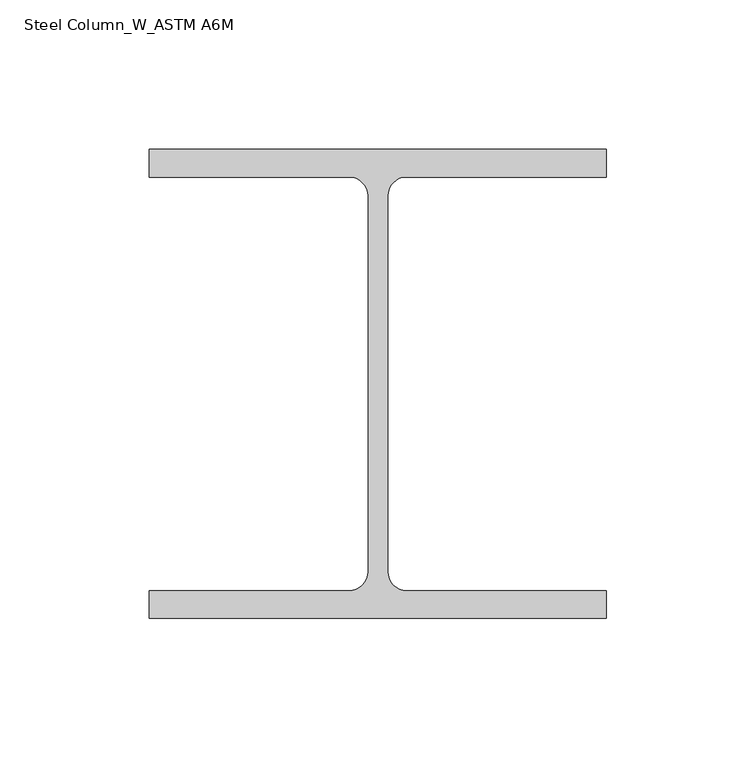
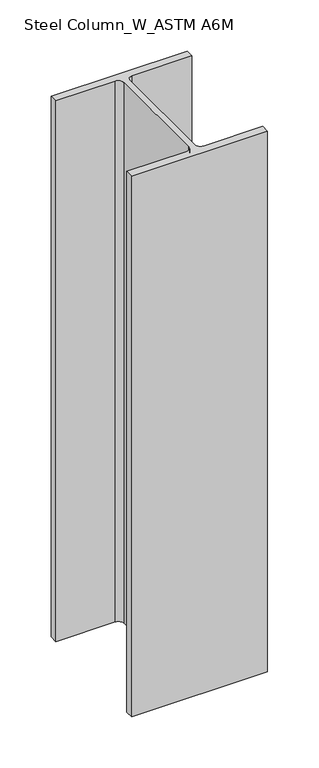
"""IFC4 building model written with IfcOpenShell, lengths in millimetres: column geometry, Steel Column_W_ASTM A6M : H_SC_AR_S01_W150x29.8_P1."""

import ifcopenshell
import ifcopenshell.guid

model = None  # the IFC model being written
_history = None  # IfcOwnerHistory: only IFC2X3 demands one
_inside = {}  # id of a spatial element -> (the spatial element, [elements in it])
_under = {}  # id of a project, library or spatial element -> (it, [spatial elements below it])
_declared = {}  # id of a project -> (the project, [libraries it declares])
_typed = {}  # id of a type object -> (the type object, [elements of that type])
_made_of = {}  # id of a material, layer set ... -> (it, [elements and type objects made of it])


def new_model(schema):
    """Start an empty IFC model of exactly this schema.

    Asked for "IFC4X3", IfcOpenShell would pick the latest addendum, in which some entities
    have other attributes; the version numbers below select the first issue.
    IFC2X3 requires an IfcOwnerHistory on every rooted entity: one is made here for all.
    """
    global model, _history
    if schema == "IFC4X3":
        model = ifcopenshell.file(schema_version=(4, 3, 0, 0))
    else:
        model = ifcopenshell.file(schema=schema)
    _inside.clear()
    _under.clear()
    _declared.clear()
    _typed.clear()
    _made_of.clear()
    _history = None
    if model.schema == "IFC2X3":
        org = make("IfcOrganization", Name="unknown")
        user = make(
            "IfcPersonAndOrganization",
            ThePerson=make("IfcPerson", FamilyName="unknown"),
            TheOrganization=org,
        )
        app = make(
            "IfcApplication",
            ApplicationDeveloper=org,
            Version="unknown",
            ApplicationFullName="unknown",
            ApplicationIdentifier="unknown",
        )
        _history = make(
            "IfcOwnerHistory",
            OwningUser=user,
            OwningApplication=app,
            ChangeAction="ADDED",
            CreationDate=0,
        )
    return model


def make(cls, **values):
    """One entity of the class cls with the attributes given. An attribute that is None is left unset."""
    return model.create_entity(
        cls, **{name: value for name, value in values.items() if value is not None}
    )


def rooted(cls, **values):
    """An entity with a GlobalId (a new one), such as an element, a storey or a relation."""
    return make(cls, GlobalId=ifcopenshell.guid.new(), OwnerHistory=_history, **values)


def si_unit(unit_type, name, prefix=None):
    """IfcSIUnit, for example si_unit("LENGTHUNIT", "METRE", prefix="MILLI")."""
    return make("IfcSIUnit", UnitType=unit_type, Prefix=prefix, Name=name)


def assignment(units):
    """IfcUnitAssignment: the units of a project."""
    return None if units is None else make("IfcUnitAssignment", Units=units)


def point(xyz):
    """IfcCartesianPoint."""
    return None if xyz is None else make("IfcCartesianPoint", Coordinates=xyz)


def direction(xyz):
    """IfcDirection."""
    return None if xyz is None else make("IfcDirection", DirectionRatios=xyz)


def frame(location, z_axis=None, x_axis=None):
    """IfcAxis2Placement3D, a coordinate frame: its origin and axes. An axis left out is left unset."""
    return make(
        "IfcAxis2Placement3D",
        Location=point(location),
        Axis=direction(z_axis),
        RefDirection=direction(x_axis),
    )


def frame_2d(location, x_axis=None):
    """IfcAxis2Placement2D, a coordinate frame in the plane: its origin and x axis."""
    return make(
        "IfcAxis2Placement2D", Location=point(location), RefDirection=direction(x_axis)
    )


def origin():
    """The frame at (0, 0, 0) with its axes left unset."""
    return frame((0.0, 0.0, 0.0))


def place(relative_to, where):
    """IfcLocalPlacement: puts the frame where relative to a parent placement (None: the world)."""
    return make(
        "IfcLocalPlacement", PlacementRelTo=relative_to, RelativePlacement=where
    )


def context(
    kind, dimensions, precision=None, world=None, true_north=None, identifier=None
):
    """IfcGeometricRepresentationContext, for example the 3D "Model" context."""
    return make(
        "IfcGeometricRepresentationContext",
        ContextIdentifier=identifier,
        ContextType=kind,
        CoordinateSpaceDimension=dimensions,
        Precision=precision,
        WorldCoordinateSystem=world,
        TrueNorth=true_north,
    )


def project(units=None, contexts=None):
    """IfcProject with its units and contexts."""
    return rooted(
        "IfcProject",
        Name="project",
        RepresentationContexts=contexts,
        UnitsInContext=assignment(units),
    )


def spatial(cls, under=None, at=None, **own):
    """A site, building, storey or space (cls), placed at a placement, below another one or the project."""
    s = rooted(cls, ObjectPlacement=at, **own)
    if under is not None:
        _under.setdefault(under.id(), (under, []))[1].append(s)
    return s


def polyline(points):
    """IfcPolyline through the points."""
    return make("IfcPolyline", Points=[point(p) for p in points])


def circle_curve(where, radius):
    """IfcCircle in the frame where."""
    return make("IfcCircle", Position=where, Radius=radius)


def trimmed(basis, trim1, trim2, sense, master):
    """IfcTrimmedCurve: the piece of a basis curve between two trims."""
    return make(
        "IfcTrimmedCurve",
        BasisCurve=basis,
        Trim1=trim1,
        Trim2=trim2,
        SenseAgreement=sense,
        MasterRepresentation=master,
    )


def segment(curve, same_sense, transition):
    """IfcCompositeCurveSegment."""
    return make(
        "IfcCompositeCurveSegment",
        Transition=transition,
        SameSense=same_sense,
        ParentCurve=curve,
    )


def composite_curve(segments, self_intersect=None):
    """IfcCompositeCurve: segments joined end to end."""
    return make("IfcCompositeCurve", Segments=segments, SelfIntersect=self_intersect)


def outline(outer, holes=None, kind="AREA"):
    """IfcArbitraryClosedProfileDef: a profile drawn as a closed curve; with holes, ...WithVoids."""
    if holes is None:
        return make("IfcArbitraryClosedProfileDef", ProfileType=kind, OuterCurve=outer)
    return make(
        "IfcArbitraryProfileDefWithVoids",
        ProfileType=kind,
        OuterCurve=outer,
        InnerCurves=holes,
    )


def extrude(swept, where, along, depth):
    """IfcExtrudedAreaSolid: the profile swept, set in the frame where, extruded along a direction by depth."""
    return make(
        "IfcExtrudedAreaSolid",
        SweptArea=swept,
        Position=where,
        ExtrudedDirection=direction(along),
        Depth=depth,
    )


def shape(context_of_items, identifier, shape_type, items):
    """IfcShapeRepresentation: the items that make up one representation, for example the "Body"."""
    return make(
        "IfcShapeRepresentation",
        ContextOfItems=context_of_items,
        RepresentationIdentifier=identifier,
        RepresentationType=shape_type,
        Items=items,
    )


def source(mapping_origin, context_of_items, identifier, shape_type, items):
    """IfcRepresentationMap: a shape defined once, which mapped items show again and again."""
    return make(
        "IfcRepresentationMap",
        MappingOrigin=mapping_origin,
        MappedRepresentation=shape(context_of_items, identifier, shape_type, items),
    )


def transform(
    local_origin,
    x_axis=None,
    y_axis=None,
    z_axis=None,
    scale=None,
    scale2=None,
    scale3=None,
    uniform=True,
):
    """IfcCartesianTransformationOperator3D, or its non-uniform kind. x_axis, y_axis, z_axis: its Axis1, 2, 3."""
    if uniform:
        return make(
            "IfcCartesianTransformationOperator3D",
            Axis1=direction(x_axis),
            Axis2=direction(y_axis),
            LocalOrigin=point(local_origin),
            Scale=scale,
            Axis3=direction(z_axis),
        )
    return make(
        "IfcCartesianTransformationOperator3DnonUniform",
        Axis1=direction(x_axis),
        Axis2=direction(y_axis),
        LocalOrigin=point(local_origin),
        Scale=scale,
        Axis3=direction(z_axis),
        Scale2=scale2,
        Scale3=scale3,
    )


def mapped(mapping_source, mapping_target):
    """IfcMappedItem: shows the shape of a source again, moved by a transform."""
    return make(
        "IfcMappedItem", MappingSource=mapping_source, MappingTarget=mapping_target
    )


def made_of(thing, what):
    """Note that an element or type object is made of a material, layer set ...; save() writes the relation."""
    if what is not None:
        _made_of.setdefault(what.id(), (what, []))[1].append(thing)
    return thing


def element(
    cls,
    number,
    at=None,
    inside=None,
    cuts=None,
    type_object=None,
    material=None,
    context=None,
    identifier="Body",
    shape_type=None,
    held_by="IfcProductDefinitionShape",
    body=None,
    shapes=None,
    **own,
):
    """One element of the class cls, such as IfcWall. Its Tag is "e" and its number.

    at: its placement. inside: the storey or other place that contains it. cuts: it is an
    opening in that element (IfcRelVoidsElement). A single representation is given by context,
    identifier, shape_type and body (its items); several are given by shapes. held_by: the class
    of the entity that holds the representations. save() writes the other relations.
    """
    e = rooted(cls, Tag="e%d" % number, ObjectPlacement=at, **own)
    if body is not None:
        shapes = [shape(context, identifier, shape_type, body)]
    if shapes is not None:
        e.Representation = make(held_by, Representations=shapes)
    if inside is not None:
        _inside.setdefault(inside.id(), (inside, []))[1].append(e)
    if cuts is not None:
        rooted(
            "IfcRelVoidsElement", RelatingBuildingElement=cuts, RelatedOpeningElement=e
        )
    if type_object is not None:
        _typed.setdefault(type_object.id(), (type_object, []))[1].append(e)
    return made_of(e, material)


def aggregate(whole, parts):
    """IfcRelAggregates: a whole, such as a stair, and the parts it consists of."""
    return rooted("IfcRelAggregates", RelatingObject=whole, RelatedObjects=parts)


def save(model, path):
    """Write the relations noted so far, then the file.

    IfcRelAggregates (storeys below a building ...), IfcRelContainedInSpatialStructure (elements
    in a storey), IfcRelDefinesByType, IfcRelAssociatesMaterial and IfcRelDeclares: one each for
    every whole, place, type object, material and project.
    """
    for whole, parts in _under.values():
        aggregate(whole, parts)
    for where, things in _inside.values():
        rooted(
            "IfcRelContainedInSpatialStructure",
            RelatedElements=things,
            RelatingStructure=where,
        )
    for kind, things in _typed.values():
        rooted("IfcRelDefinesByType", RelatedObjects=things, RelatingType=kind)
    for what, things in _made_of.values():
        rooted("IfcRelAssociatesMaterial", RelatedObjects=things, RelatingMaterial=what)
    for by, libraries in _declared.values():
        rooted("IfcRelDeclares", RelatingContext=by, RelatedDefinitions=libraries)
    model.write(path)


def steel_column_w_astm_a6m_853d7517(model_context):
    return source(origin(), model_context, "Body", "SweptSolid", [
        extrude(outline(composite_curve([segment(polyline([(76.5, 78.5), (76.5, 69.23), (9.63, 69.23)]), True, "CONTINUOUS"), segment(trimmed(circle_curve(frame_2d((9.63, 62.9)), 6.33), [point((9.63, 69.23))], [point((3.3, 62.9))], True, "CARTESIAN"), True, "CONTINUOUS"), segment(polyline([(3.3, 62.9), (3.3, -62.9)]), True, "CONTINUOUS"), segment(trimmed(circle_curve(frame_2d((9.63, -62.9)), 6.33), [point((3.3, -62.9))], [point((9.63, -69.23))], True, "CARTESIAN"), True, "CONTINUOUS"), segment(polyline([(9.63, -69.23), (76.5, -69.23), (76.5, -78.5), (-76.5, -78.5), (-76.5, -69.23), (-9.63, -69.23)]), True, "CONTINUOUS"), segment(trimmed(circle_curve(frame_2d((-9.63, -62.9)), 6.33), [point((-9.63, -69.23))], [point((-3.3, -62.9))], True, "CARTESIAN"), True, "CONTINUOUS"), segment(polyline([(-3.3, -62.9), (-3.3, 62.9)]), True, "CONTINUOUS"), segment(trimmed(circle_curve(frame_2d((-9.63, 62.9)), 6.33), [point((-3.3, 62.9))], [point((-9.63, 69.23))], True, "CARTESIAN"), True, "CONTINUOUS"), segment(polyline([(-9.63, 69.23), (-76.5, 69.23), (-76.5, 78.5), (76.5, 78.5)]), True, "CONTINUOUS")], self_intersect=False)), frame((0.0, 0.0, 1519.8243501), z_axis=(0.0, 0.0, 1.0), x_axis=(1.0, 0.0, 0.0)), (0.0, 0.0, 1.0), 644.0),
    ])


if __name__ == "__main__":
    model = new_model("IFC4")
    model_context = context("Model", 3, world=origin())
    ifc_project = project(units=[si_unit("LENGTHUNIT", "METRE", prefix="MILLI")], contexts=[model_context])
    site = spatial("IfcSite", under=ifc_project)
    building = spatial("IfcBuilding", under=site)
    placement = place(None, origin())
    steel_column_w_astm_a6m_shape = steel_column_w_astm_a6m_853d7517(model_context)
    element("IfcColumn", 1, ObjectType="Steel Column_W_ASTM A6M : H_SC_AR_S01_W150x29.8_P1", at=placement, inside=building, context=model_context, shape_type="MappedRepresentation", body=[
        mapped(steel_column_w_astm_a6m_shape, transform((0.0, 0.0, 0.0), x_axis=(1.0, 0.0, 0.0), y_axis=(0.0, 1.0, 0.0), z_axis=(0.0, 0.0, 1.0))),
    ])
    save(model, "model.ifc")

# Revit data of these elements
# Type "Steel Column_W_ASTM A6M : H_SC_AR_S01_W150x29.8_P1"
#   Section Name Key = "W6x20"
#   Width = 15.3 cm
#   Web Thickness = 0.66 cm
#   Web Fillet = 0.633 cm
#   Warping Constant = 30300.0 cm⁶
#   Torsional Moment of Inertia = 9.99 cm⁴
#   Section Area = 37.9 cm²
#   Plastic Modulus weak axis = 110.0 cm³
#   Plastic Modulus strong axis = 246.0 cm³
#   Perimeter = 0.902 m²/m
#   Nominal Weight = 29.80 kgf/m
#   Moment of Inertia weak axis = 554.00 cm⁴
#   Moment of Inertia strong axis = 1720.00 cm⁴
#   Height = 15.7 cm
#   Flange Thickness = 0.927 cm
#   Elastic Modulus weak axis = 72.3 cm³
#   Elastic Modulus strong axis = 220.0 cm³
#   Centroid Vertical = 7.85 cm
#   Centroid Horizontal = 7.65 cm
#   Structural Material [instance default] = Steel, 45-345
#   Bolt Spacing = 0
#   Assembly Code = ""
# Element 1 (IfcColumn, "Steel Column_W_ASTM A6M : H_SC_AR_S01_W150x29.8_P1")
#   Structural Material = none
# Materials
#   "Steel, 45-345": class "Metal", colour RGB 189 187 185, transparency 0, Description = "Steel 345 MPa", Cost = 0
